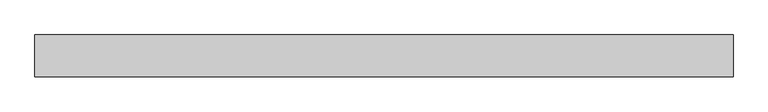
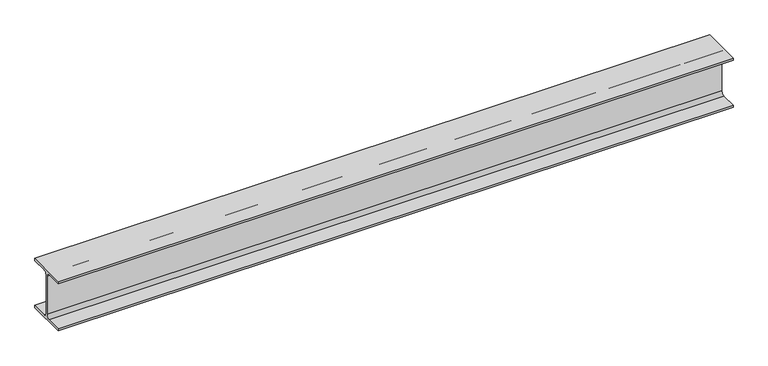
"""IFC4 building model written with IfcOpenShell, lengths in millimetres: beam geometry, 0912_Steel Framing_H-KSD3502 : H_SB_ASB_H-194x150x6x9."""

from ifc_helpers import new_model, si_unit, point, frame, frame_2d, origin, place, context, project, spatial, polyline, circle_curve, trimmed, segment, composite_curve, outline, extrude, source, transform, mapped, element, save


def beam_dc8ab3e4(model_context):
    return source(origin(), model_context, "Body", "SweptSolid", [
        extrude(outline(composite_curve([segment(polyline([(-75.0, -88.0), (-16.0, -88.0)]), True, "CONTINUOUS"), segment(trimmed(circle_curve(frame_2d((-16.0, -75.0)), 13.0), [point((-16.0, -88.0))], [point((-3.0, -75.0))], True, "CARTESIAN"), True, "CONTINUOUS"), segment(polyline([(-3.0, -75.0), (-3.0, 75.0)]), True, "CONTINUOUS"), segment(trimmed(circle_curve(frame_2d((-16.0, 75.0)), 13.0), [point((-3.0, 75.0))], [point((-16.0, 88.0))], True, "CARTESIAN"), True, "CONTINUOUS"), segment(polyline([(-16.0, 88.0), (-75.0, 88.0), (-75.0, 97.0), (75.0, 97.0), (75.0, 88.0), (16.0, 88.0)]), True, "CONTINUOUS"), segment(trimmed(circle_curve(frame_2d((16.0, 75.0)), 13.0), [point((16.0, 88.0))], [point((3.0, 75.0))], True, "CARTESIAN"), True, "CONTINUOUS"), segment(polyline([(3.0, 75.0), (3.0, -75.0)]), True, "CONTINUOUS"), segment(trimmed(circle_curve(frame_2d((16.0, -75.0)), 13.0), [point((3.0, -75.0))], [point((16.0, -88.0))], True, "CARTESIAN"), True, "CONTINUOUS"), segment(polyline([(16.0, -88.0), (75.0, -88.0), (75.0, -97.0), (-75.0, -97.0), (-75.0, -88.0)]), True, "CONTINUOUS")], self_intersect=False)), frame((-1130.4393685, 0.0, 0.0), z_axis=(1.0, 0.0, 0.0), x_axis=(0.0, 1.0, 0.0)), (0.0, 0.0, 1.0), 2507.5454037),
    ])


if __name__ == "__main__":
    model = new_model("IFC4")
    model_context = context("Model", 3, world=origin())
    ifc_project = project(units=[si_unit("LENGTHUNIT", "METRE", prefix="MILLI")], contexts=[model_context])
    site = spatial("IfcSite", under=ifc_project)
    building = spatial("IfcBuilding", under=site)
    placement = place(None, origin())
    beam_shape = beam_dc8ab3e4(model_context)
    element("IfcBeam", 1, ObjectType="0912_Steel Framing_H-KSD3502 : H_SB_ASB_H-194x150x6x9", at=placement, inside=building, context=model_context, shape_type="MappedRepresentation", body=[
        mapped(beam_shape, transform((0.0, 0.0, 0.0), x_axis=(1.0, 0.0, 0.0), y_axis=(0.0, 1.0, 0.0), z_axis=(0.0, 0.0, 1.0))),
    ])
    save(model, "model.ifc")

# Revit data of these elements
# Type "0912_Steel Framing_H-KSD3502 : H_SB_ASB_H-194x150x6x9"
#   H_WM Code_1 = "S01AA002-00001 | Main Steel Structure Fabrication Work | Shelter/Building | Medium Steel - Standard (90KG/M>Weight≥30KG/M) | Material: (   )"
#   H_WM Code_2 = "S03AA028-00001 | Main Steel Structure Erection Work | Shelter/Building | Medium Steel (90KG/M>Weight≥30KG/M) | Material: (   )"
#   H_WM Code_3 = "S01AA010-00001 | Main Steel Structure Fabrication Work | Shelter/Building | Steel Painting/Coating | for Non-Fireproofed Steel Surface, Surface Preparation, Primer, Second & Final Coat | Material: (   )"
#   H_Q'ty Cal Type Tag = "SB-Q2"
#   Width = 15.0 cm
#   Web Thickness = 0.6 cm
#   Web Fillet = 1.3 cm
#   Warping Constant = 43316.0 cm⁶
#   W = 0
#   Torsional Moment of Inertia = 8.622 cm⁴
#   Section Area = 39.01 cm²
#   Plastic Modulus weak axis = 104.0 cm³
#   Plastic Modulus strong axis = 309.0 cm³
#   Perimeter = 0.95 m²/m
#   Nominal Weight = 30.60 kgf/m
#   Moment of Inertia weak axis = 507.00 cm⁴
#   Moment of Inertia strong axis = 2690.00 cm⁴
#   Height = 19.4 cm
#   Flange Thickness = 0.9 cm
#   Elastic Modulus weak axis = 67.6 cm³
#   Elastic Modulus strong axis = 277.0 cm³
#   Centroid Vertical = 9.7 cm
#   Centroid Horizontal = 7.5 cm
#   Ix = 26900000
#   Length [instance default] = 1.5240 m
#   Zx = 309000
#   b = 0.1500 m
#   h = 0.1940 m
#   r = 0.0130 m
#   s = 0.0060 m
#   t = 0.0090 m
#   A = 0.003901 m²
#   Structural Material [instance default] = Steel, 45-345
#   Assembly Code = ""
# Element 1 (IfcBeam, "0912_Steel Framing_H-KSD3502 : H_SB_ASB_H-194x150x6x9")
#   Structural Material = none
# Materials
#   "Steel, 45-345": class "Metal", colour RGB 189 187 185, transparency 0, Description = "Steel 345 MPa", Cost = 0
